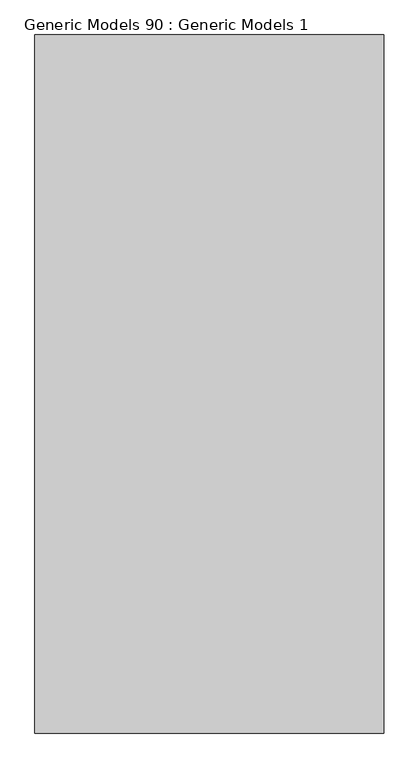
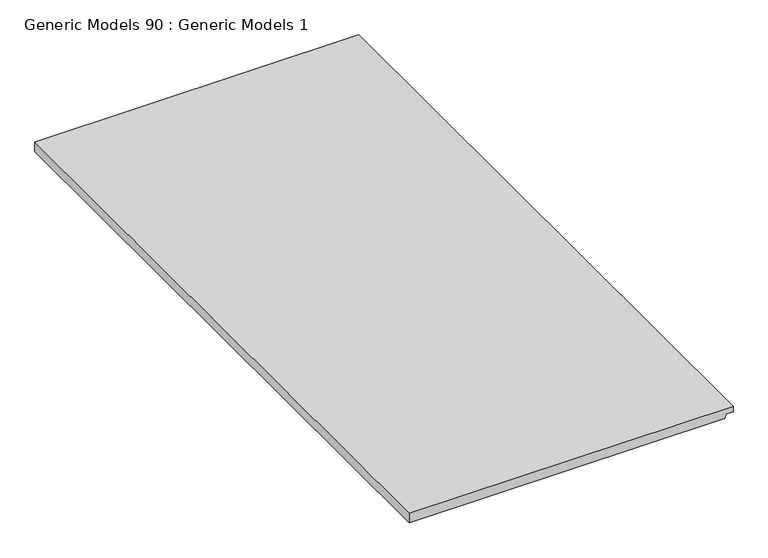
"""IFC4 building model written with IfcOpenShell, lengths in millimetres: proxy geometry, Generic Models 90 : Generic Models 1."""

from ifc_helpers import new_model, si_unit, frame, origin, place, context, project, spatial, polyline, outline, extrude, source, transform, mapped, element, save


def generic_models_90_generic_models_1_e41f1d4b(model_context):
    return source(origin(), model_context, "Body", "SweptSolid", [
        extrude(outline(polyline([(2281.1808399, 49662.5798593), (2281.1808399, 49052.9798593), (2262.1308399, 49052.9798593), (2262.1308399, 49646.9908455), (2270.0683399, 49649.8798593), (2270.0683399, 49662.5798593), (2281.1808399, 49662.5798593)])), frame((0.0, 0.0, 0.0), z_axis=(0.0, 1.0, 0.0), x_axis=(0.0, 0.0, 1.0)), (0.0, 0.0, 1.0), 1219.2),
    ])


if __name__ == "__main__":
    model = new_model("IFC4")
    model_context = context("Model", 3, world=origin())
    ifc_project = project(units=[si_unit("LENGTHUNIT", "METRE", prefix="MILLI")], contexts=[model_context])
    site = spatial("IfcSite", under=ifc_project)
    building = spatial("IfcBuilding", under=site)
    placement = place(None, origin())
    generic_models_90_generic_models_1_shape = generic_models_90_generic_models_1_e41f1d4b(model_context)
    element("IfcBuildingElementProxy", 1, Name="Generic Models 90 : Generic Models 1", ObjectType="Generic Models 90 : Generic Models 1", at=placement, inside=building, context=model_context, shape_type="MappedRepresentation", body=[
        mapped(generic_models_90_generic_models_1_shape, transform((0.0, 0.0, 0.0), x_axis=(1.0, 0.0, 0.0), y_axis=(0.0, 1.0, 0.0), z_axis=(0.0, 0.0, 1.0))),
    ])
    save(model, "model.ifc")

# Revit data of these elements
# Element 1 (IfcBuildingElementProxy, "Generic Models 90 : Generic Models 1")
#   Materials on its faces: "CEILING AS SCHEDULED"
# Materials
#   "CEILING AS SCHEDULED": class "Generic", colour RGB 255 255 255, transparency 0, Cost = 0
